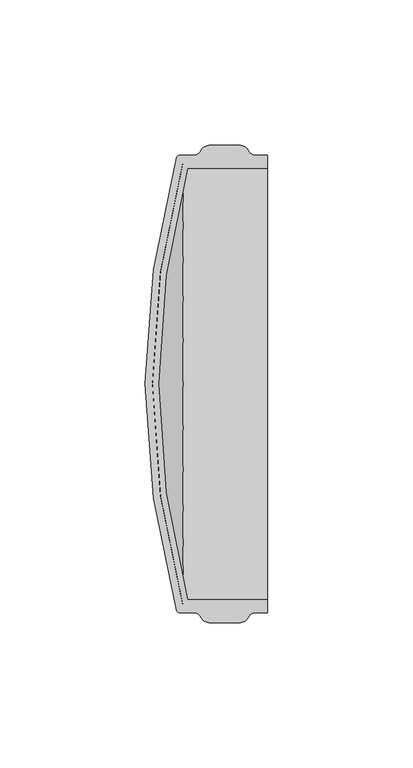
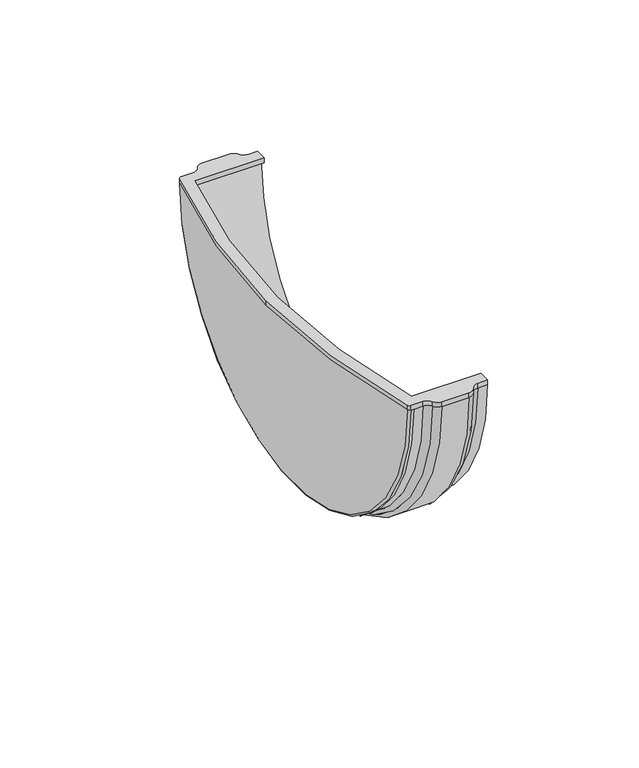
"""IFC4 building model written with IfcOpenShell, lengths in millimetres: proxy geometry, ↩ Заглушка желоба : ↩ Заглушка желоба."""

from ifc_helpers import new_model, si_unit, point, frame, origin, place, context, project, spatial, polyline, circle_curve, ellipse_curve, trimmed, source, transform, mapped, element, save
from ifc_brep_helpers import plane_surface, cylinder_surface, revolved_surface, advanced_brep


def generic_models_0d5aeb62(model_context):
    return source(origin(), model_context, "Body", "AdvancedBrep", [
        advanced_brep(
        [(-25.5074023, -78.6, 0.0), (-29.0, -78.6, 0.0), (-29.0, 78.6, 0.0), (-25.5074023, 78.6, 0.0), (-22.8037012, 80.3, 0.0), (-22.8037012, -80.3, 0.0), (-20.1, 82.0, 0.0), (-20.1, -82.0, 0.0), (-9.3443413, 82.0, 0.0), (-9.3443413, -82.0, 0.0), (-6.6406401, 80.3, 0.0), (-6.6406401, -80.3, 0.0), (-3.936939, 78.6, 0.0), (-3.936939, -78.6, 0.0), (-0.0443413, 78.6, 0.0), (-0.0443413, -78.6, 0.0), (-0.0443413, 78.6, 2.0), (-0.0443413, 74.1, 2.0), (-0.0443413, 74.1, 0.0), (-0.0443413, 76.1, 0.0), (-0.0443413, -76.1, 0.0), (-0.0443413, -74.1, 0.0), (-0.0443413, -74.1, 2.0), (-0.0443413, -78.6, 2.0), (-29.0, 76.1, 0.0), (-29.0, -76.1, 0.0), (-31.2572877, -77.8330313, 0.0), (-42.0295138, 0.0, 0.0), (-31.2572877, 77.8330313, 0.0), (-30.2504109, 78.6, 0.0), (-30.2504109, -78.6, 0.0), (-39.5258282, 0.0, 0.0), (-27.4693868, -74.1, 2.0), (-37.5257643, 0.0, 2.0), (-27.4693868, 74.1, 2.0), (-3.936939, 78.6, 2.0), (-6.6406401, 80.3, 2.0), (-9.3443413, 82.0, 2.0), (-20.1, 82.0, 2.0), (-22.8037012, 80.3, 2.0), (-25.5074023, 78.6, 2.0), (-30.2504109, 78.6, 2.0), (-31.2572877, 77.8330313, 2.0), (-42.0295138, 0.0, 2.0), (-31.2572877, -77.8330313, 2.0), (-30.2504109, -78.6, 2.0), (-25.5074023, -78.6, 2.0), (-22.8037012, -80.3, 2.0), (-20.1, -82.0, 2.0), (-9.3443413, -82.0, 2.0), (-6.6406401, -80.3, 2.0), (-3.936939, -78.6, 2.0), (-27.4693868, 74.1, 0.0), (-37.5257643, 0.0, 0.0), (-27.4693868, -74.1, 0.0)],
        [
            (0, 1),
            (1, 2, circle_curve(frame((-29.0, 0.0, 0.0), z_axis=(1.0, 0.0, 0.0), x_axis=(0.0, 1.0, 0.0)), 78.6)),
            (2, 3),
            (3, 0, circle_curve(frame((-25.5074023, 0.0, 0.0), z_axis=(-1.0, 0.0, 0.0), x_axis=(0.0, 1.0, 0.0)), 78.6)),
            (3, 4, circle_curve(frame((-25.5074023, 81.6, 0.0), z_axis=(0.0, 0.0, 1.0), x_axis=(1.0, 0.0, 0.0)), 3.0)),
            (4, 5, circle_curve(frame((-22.8037012, 0.0, 0.0), z_axis=(-1.0, 0.0, 0.0), x_axis=(0.0, 1.0, 0.0)), 80.3)),
            (5, 0, circle_curve(frame((-25.5074023, -81.6, 0.0), z_axis=(0.0, 0.0, 1.0), x_axis=(1.0, 0.0, 0.0)), 3.0)),
            (4, 6, circle_curve(frame((-20.1, 79.0, 0.0), z_axis=(0.0, 0.0, -1.0), x_axis=(1.0, 0.0, 0.0)), 3.0)),
            (6, 7, circle_curve(frame((-20.1, 0.0, 0.0), z_axis=(-1.0, 0.0, 0.0), x_axis=(0.0, 1.0, 0.0)), 82.0)),
            (7, 5, circle_curve(frame((-20.1, -79.0, 0.0), z_axis=(0.0, 0.0, -1.0), x_axis=(1.0, 0.0, 0.0)), 3.0)),
            (6, 8),
            (8, 9, circle_curve(frame((-9.3443413, 0.0, 0.0), z_axis=(-1.0, 0.0, 0.0), x_axis=(0.0, 1.0, 0.0)), 82.0)),
            (9, 7),
            (8, 10, circle_curve(frame((-9.3443413, 79.0, 0.0), z_axis=(0.0, 0.0, -1.0), x_axis=(-1.0, 0.0, 0.0)), 3.0)),
            (10, 11, circle_curve(frame((-6.6406401, 0.0, 0.0), z_axis=(-1.0, 0.0, 0.0), x_axis=(0.0, 1.0, 0.0)), 80.3)),
            (11, 9, circle_curve(frame((-9.3443413, -79.0, 0.0), z_axis=(0.0, 0.0, -1.0), x_axis=(-1.0, 0.0, 0.0)), 3.0)),
            (10, 12, circle_curve(frame((-3.936939, 81.6, 0.0), z_axis=(0.0, 0.0, 1.0), x_axis=(-1.0, 0.0, 0.0)), 3.0)),
            (12, 13, circle_curve(frame((-3.936939, 0.0, 0.0), z_axis=(-1.0, 0.0, 0.0), x_axis=(0.0, 1.0, 0.0)), 78.6)),
            (13, 11, circle_curve(frame((-3.936939, -81.6, 0.0), z_axis=(0.0, 0.0, 1.0), x_axis=(-1.0, 0.0, 0.0)), 3.0)),
            (12, 14),
            (14, 15, circle_curve(frame((-0.0443413, 0.0, 0.0), z_axis=(-1.0, 0.0, 0.0), x_axis=(0.0, 1.0, 0.0)), 78.6)),
            (15, 13),
            (14, 16),
            (16, 17),
            (17, 18),
            (18, 19),
            (19, 20, circle_curve(frame((-0.0443413, 0.0, 0.0), z_axis=(-1.0, 0.0, 0.0), x_axis=(0.0, 1.0, 0.0)), 76.1)),
            (20, 21),
            (21, 22),
            (22, 23),
            (23, 15),
            (19, 24),
            (24, 25, circle_curve(frame((-29.0, 0.0, 0.0), z_axis=(-1.0, 0.0, 0.0), x_axis=(0.0, 1.0, 0.0)), 76.1)),
            (25, 20),
            (26, 27, circle_curve(frame((257.964734, 1.8577595, 0.0), z_axis=(0.0, 0.0, -1.0), x_axis=(1.0, 0.0, 0.0)), 300.0)),
            (27, 28, circle_curve(frame((257.964734, -1.8577595, 0.0), z_axis=(0.0, 0.0, -1.0), x_axis=(1.0, 0.0, 0.0)), 300.0)),
            (28, 26, circle_curve(frame((-31.2572877, 0.0, 0.0), z_axis=(-1.0, 0.0, 0.0), x_axis=(0.0, 1.0, 0.0)), 77.8330313)),
            (28, 29, circle_curve(frame((-30.2504109, 77.5556015, 0.0), z_axis=(0.0, 0.0, -1.0), x_axis=(1.0, 0.0, 0.0)), 1.0443985)),
            (29, 30, circle_curve(frame((-30.2504109, 0.0, 0.0), z_axis=(-1.0, 0.0, 0.0), x_axis=(0.0, 1.0, 0.0)), 78.6)),
            (30, 26, circle_curve(frame((-30.2504109, -77.5556015, 0.0), z_axis=(0.0, 0.0, -1.0), x_axis=(1.0, 0.0, 0.0)), 1.0443985)),
            (29, 2),
            (1, 30),
            (24, 31, circle_curve(frame((257.964734, -2.3696848, 0.0), z_axis=(0.0, 0.0, 1.0), x_axis=(1.0, 0.0, 0.0)), 297.5)),
            (31, 25, circle_curve(frame((257.964734, 2.3696848, 0.0), z_axis=(0.0, 0.0, 1.0), x_axis=(1.0, 0.0, 0.0)), 297.5)),
            (22, 32),
            (32, 33, circle_curve(frame((257.964734, 2.3696848, 2.0), z_axis=(0.0, 0.0, -1.0), x_axis=(1.0, 0.0, 0.0)), 295.5)),
            (33, 34, circle_curve(frame((257.964734, -2.3696848, 2.0), z_axis=(0.0, 0.0, -1.0), x_axis=(1.0, 0.0, 0.0)), 295.5)),
            (34, 17),
            (16, 35),
            (35, 36, circle_curve(frame((-3.936939, 81.6, 2.0), z_axis=(0.0, 0.0, -1.0), x_axis=(1.0, 0.0, 0.0)), 3.0)),
            (36, 37, circle_curve(frame((-9.3443413, 79.0, 2.0), z_axis=(0.0, 0.0, 1.0), x_axis=(1.0, 0.0, 0.0)), 3.0)),
            (37, 38),
            (38, 39, circle_curve(frame((-20.1, 79.0, 2.0), z_axis=(0.0, 0.0, 1.0), x_axis=(1.0, 0.0, 0.0)), 3.0)),
            (39, 40, circle_curve(frame((-25.5074023, 81.6, 2.0), z_axis=(0.0, 0.0, -1.0), x_axis=(1.0, 0.0, 0.0)), 3.0)),
            (40, 41),
            (41, 42, circle_curve(frame((-30.2504109, 77.5556015, 2.0), z_axis=(0.0, 0.0, 1.0), x_axis=(1.0, 0.0, 0.0)), 1.0443985)),
            (42, 43, circle_curve(frame((257.964734, -1.8577595, 2.0), z_axis=(0.0, 0.0, 1.0), x_axis=(1.0, 0.0, 0.0)), 300.0)),
            (43, 44, circle_curve(frame((257.964734, 1.8577595, 2.0), z_axis=(0.0, 0.0, 1.0), x_axis=(1.0, 0.0, 0.0)), 300.0)),
            (44, 45, circle_curve(frame((-30.2504109, -77.5556015, 2.0), z_axis=(0.0, 0.0, 1.0), x_axis=(1.0, 0.0, 0.0)), 1.0443985)),
            (45, 46),
            (46, 47, circle_curve(frame((-25.5074023, -81.6, 2.0), z_axis=(0.0, 0.0, -1.0), x_axis=(1.0, 0.0, 0.0)), 3.0)),
            (47, 48, circle_curve(frame((-20.1, -79.0, 2.0), z_axis=(0.0, 0.0, 1.0), x_axis=(1.0, 0.0, 0.0)), 3.0)),
            (48, 49),
            (49, 50, circle_curve(frame((-9.3443413, -79.0, 2.0), z_axis=(0.0, 0.0, 1.0), x_axis=(1.0, 0.0, 0.0)), 3.0)),
            (50, 51, circle_curve(frame((-3.936939, -81.6, 2.0), z_axis=(0.0, 0.0, -1.0), x_axis=(1.0, 0.0, 0.0)), 3.0)),
            (51, 23),
            (18, 52),
            (52, 53, circle_curve(frame((257.964734, -2.3696848, 0.0), z_axis=(0.0, 0.0, 1.0), x_axis=(1.0, 0.0, 0.0)), 295.5)),
            (53, 54, circle_curve(frame((257.964734, 2.3696848, 0.0), z_axis=(0.0, 0.0, 1.0), x_axis=(1.0, 0.0, 0.0)), 295.5)),
            (54, 21),
            (51, 13),
            (50, 11),
            (49, 9),
            (48, 7),
            (47, 5),
            (46, 0),
            (45, 30),
            (44, 26),
            (43, 27),
            (42, 28),
            (41, 29),
            (40, 3),
            (39, 4),
            (38, 6),
            (37, 8),
            (36, 10),
            (35, 12),
            (34, 52),
            (33, 53),
            (32, 54),
        ],
        [
            cylinder_surface(frame((-14.7221706, 0.0, 0.0), z_axis=(1.0, 0.0, 0.0), x_axis=(0.0, 1.0, 0.0)), 78.6),
            revolved_surface(trimmed(ellipse_curve(frame((-25.5074023, 81.6, 0.0), z_axis=(0.0, 0.0, 1.0), x_axis=(1.0, 0.0, 0.0)), 3.0, 3.0), [point((-25.5074023, 78.6, 0.0))], [point((-22.8037012, 80.3, 0.0))], True, "CARTESIAN"), (-14.7221706, 0.0, 0.0), (1.0, 0.0, 0.0)),
            revolved_surface(trimmed(ellipse_curve(frame((-20.1, 79.0, 0.0), z_axis=(0.0, 0.0, -1.0), x_axis=(1.0, 0.0, 0.0)), 3.0, 3.0), [point((-22.8037012, 80.3, 0.0))], [point((-20.1, 82.0, 0.0))], True, "CARTESIAN"), (-14.7221706, 0.0, 0.0), (1.0, 0.0, 0.0)),
            cylinder_surface(frame((-14.7221706, 0.0, 0.0), z_axis=(1.0, 0.0, 0.0), x_axis=(0.0, 1.0, 0.0)), 82.0),
            revolved_surface(trimmed(ellipse_curve(frame((-9.3443413, 79.0, 0.0), z_axis=(0.0, 0.0, -1.0), x_axis=(-1.0, 0.0, 0.0)), 3.0, 3.0), [point((-9.3443413, 82.0, 0.0))], [point((-6.6406401, 80.3, 0.0))], True, "CARTESIAN"), (-14.7221706, 0.0, 0.0), (1.0, 0.0, 0.0)),
            revolved_surface(trimmed(ellipse_curve(frame((-3.936939, 81.6, 0.0), z_axis=(0.0, 0.0, 1.0), x_axis=(-1.0, 0.0, 0.0)), 3.0, 3.0), [point((-6.6406401, 80.3, 0.0))], [point((-3.936939, 78.6, 0.0))], True, "CARTESIAN"), (-14.7221706, 0.0, 0.0), (1.0, 0.0, 0.0)),
            plane_surface(frame((-0.0443413, 0.0, 0.0), z_axis=(1.0, 0.0, 0.0), x_axis=(0.0, 1.0, 0.0))),
            revolved_surface(polyline([(-0.04434129999999925, 76.1, 0.0), (-29.0, 76.1, 0.0)]), (-14.7221706, 0.0, 0.0), (1.0, 0.0, 0.0)),
            revolved_surface(trimmed(ellipse_curve(frame((257.964734, -1.8577595, 0.0), z_axis=(0.0, 0.0, -1.0), x_axis=(1.0, 0.0, 0.0)), 300.0, 300.0), [point((-42.0295138, 0.0, 0.0))], [point((-31.2572877, 77.8330313, 0.0))], True, "CARTESIAN"), (-42.0, 0.0, 0.0), (1.0, 0.0, 0.0)),
            revolved_surface(trimmed(ellipse_curve(frame((-30.2504109, 77.5556015, 0.0), z_axis=(0.0, 0.0, -1.0), x_axis=(1.0, 0.0, 0.0)), 1.0443985, 1.0443985), [point((-31.2572877, 77.8330313, 0.0))], [point((-30.2504109, 78.6, 0.0))], True, "CARTESIAN"), (-42.0, 0.0, 0.0), (1.0, 0.0, 0.0)),
            cylinder_surface(frame((-42.0, 0.0, 0.0), z_axis=(1.0, 0.0, 0.0), x_axis=(0.0, 1.0, 0.0)), 78.6),
            revolved_surface(trimmed(ellipse_curve(frame((257.964734, -2.3696848, 0.0), z_axis=(0.0, 0.0, 1.0), x_axis=(1.0, 0.0, 0.0)), 297.5, 297.5), [point((-29.0, 76.1, 0.0))], [point((-39.5258282, 0.0, 0.0))], True, "CARTESIAN"), (-42.0, 0.0, 0.0), (1.0, 0.0, 0.0)),
            plane_surface(frame((-0.0443413, -78.6, 2.0), z_axis=(0.0, 0.0, 1.0), x_axis=(-1.0, 0.0, 0.0))),
            plane_surface(frame((-0.0443413, -78.6, 0.0), z_axis=(0.0, 0.0, -1.0), x_axis=(1.0, 0.0, 0.0))),
            plane_surface(frame((-0.0443413, -78.6, 2.0), z_axis=(0.0, -1.0, 0.0), x_axis=(0.0, 0.0, -1.0))),
            revolved_surface(polyline([(-0.9369390000000002, -81.6, 0.0), (-0.9369390000000002, -81.6, 2.0)]), (-3.936939, -81.6, 0.0), (0.0, 0.0, -1.0)),
            cylinder_surface(frame((-9.3443413, -79.0, 0.0), z_axis=(0.0, 0.0, 1.0), x_axis=(1.0, 0.0, 0.0)), 3.0),
            plane_surface(frame((-9.3443413, -82.0, 2.0), z_axis=(0.0, -1.0, 0.0), x_axis=(0.0, 0.0, -1.0))),
            cylinder_surface(frame((-20.1, -79.0, 0.0), z_axis=(0.0, 0.0, 1.0), x_axis=(1.0, 0.0, 0.0)), 3.0),
            revolved_surface(polyline([(-22.5074023, -81.6, 0.0), (-22.5074023, -81.6, 2.0)]), (-25.5074023, -81.6, 0.0), (0.0, 0.0, -1.0)),
            plane_surface(frame((-25.5074023, -78.6, 2.0), z_axis=(0.0, -1.0, 0.0), x_axis=(0.0, 0.0, -1.0))),
            cylinder_surface(frame((-30.2504109, -77.5556015, 0.0), z_axis=(0.0, 0.0, 1.0), x_axis=(1.0, 0.0, 0.0)), 1.0443985),
            cylinder_surface(frame((257.964734, 1.8577595, 0.0), z_axis=(0.0, 0.0, 1.0), x_axis=(1.0, 0.0, 0.0)), 300.0),
            cylinder_surface(frame((257.964734, -1.8577595, 0.0), z_axis=(0.0, 0.0, 1.0), x_axis=(1.0, 0.0, 0.0)), 300.0),
            cylinder_surface(frame((-30.2504109, 77.5556015, 0.0), z_axis=(0.0, 0.0, 1.0), x_axis=(1.0, 0.0, 0.0)), 1.0443985),
            plane_surface(frame((-30.2504109, 78.6, 2.0), z_axis=(0.0, 1.0, 0.0), x_axis=(0.0, 0.0, -1.0))),
            revolved_surface(polyline([(-22.5074023, 81.6, 0.0), (-22.5074023, 81.6, 2.0)]), (-25.5074023, 81.6, 0.0), (0.0, 0.0, -1.0)),
            cylinder_surface(frame((-20.1, 79.0, 0.0), z_axis=(0.0, 0.0, 1.0), x_axis=(1.0, 0.0, 0.0)), 3.0),
            plane_surface(frame((-20.1, 82.0, 2.0), z_axis=(0.0, 1.0, 0.0), x_axis=(0.0, 0.0, -1.0))),
            cylinder_surface(frame((-9.3443413, 79.0, 0.0), z_axis=(0.0, 0.0, 1.0), x_axis=(1.0, 0.0, 0.0)), 3.0),
            revolved_surface(polyline([(-0.9369390000000002, 81.6, 0.0), (-0.9369390000000002, 81.6, 2.0)]), (-3.936939, 81.6, 0.0), (0.0, 0.0, -1.0)),
            plane_surface(frame((-3.936939, 78.6, 2.0), z_axis=(0.0, 1.0, 0.0), x_axis=(0.0, 0.0, -1.0))),
            plane_surface(frame((-0.0443413, 74.1, 2.0), z_axis=(0.0, -1.0, 0.0), x_axis=(0.0, 0.0, -1.0))),
            revolved_surface(polyline([(553.464734, -2.3696848, 0.0), (553.464734, -2.3696848, 2.0)]), (257.964734, -2.3696848, 0.0), (0.0, 0.0, -1.0)),
            revolved_surface(polyline([(553.464734, 2.3696848, 0.0), (553.464734, 2.3696848, 2.0)]), (257.964734, 2.3696848, 0.0), (0.0, 0.0, -1.0)),
            plane_surface(frame((-27.4693868, -74.1, 2.0), z_axis=(0.0, 1.0, 0.0), x_axis=(0.0, 0.0, -1.0))),
        ],
        [
            (0, [[1, 2, 3, 4]]),
            (1, [[5, 6, 7, -4]]),
            (2, [[8, 9, 10, -6]]),
            (3, [[11, 12, 13, -9]]),
            (4, [[14, 15, 16, -12]]),
            (5, [[17, 18, 19, -15]]),
            (0, [[20, 21, 22, -18]]),
            (6, [[23, 24, 25, 26, 27, 28, 29, 30, 31, -21]]),
            (7, [[32, 33, 34, -27]]),
            (8, [[35, 36, 37]]),
            (9, [[38, 39, 40, -37]]),
            (10, [[41, -2, 42, -39]]),
            (11, [[43, 44, -33]]),
            (12, [[-30, 45, 46, 47, 48, -24, 49, 50, 51, 52, 53, 54, 55, 56, 57, 58, 59, 60, 61, 62, 63, 64, 65, 66]]),
            (13, [[-28, -34, -44, -43, -32, -26, 67, 68, 69, 70]]),
            (14, [[71, -22, -31, -66]]),
            (15, [[72, -19, -71, -65]]),
            (16, [[73, -16, -72, -64]]),
            (17, [[74, -13, -73, -63]]),
            (18, [[75, -10, -74, -62]]),
            (19, [[76, -7, -75, -61]]),
            (20, [[77, -42, -1, -76, -60]]),
            (21, [[78, -40, -77, -59]]),
            (22, [[79, -35, -78, -58]]),
            (23, [[80, -36, -79, -57]]),
            (24, [[81, -38, -80, -56]]),
            (25, [[82, -3, -41, -81, -55]]),
            (26, [[83, -5, -82, -54]]),
            (27, [[84, -8, -83, -53]]),
            (28, [[85, -11, -84, -52]]),
            (29, [[86, -14, -85, -51]]),
            (30, [[87, -17, -86, -50]]),
            (31, [[-23, -20, -87, -49]]),
            (32, [[88, -67, -25, -48]]),
            (33, [[89, -68, -88, -47]]),
            (34, [[90, -69, -89, -46]]),
            (35, [[-29, -70, -90, -45]]),
        ],
    ),
    ])


if __name__ == "__main__":
    model = new_model("IFC4")
    model_context = context("Model", 3, world=origin())
    ifc_project = project(units=[si_unit("LENGTHUNIT", "METRE", prefix="MILLI")], contexts=[model_context])
    site = spatial("IfcSite", under=ifc_project)
    building = spatial("IfcBuilding", under=site)
    placement = place(None, origin())
    generic_models_shape = generic_models_0d5aeb62(model_context)
    element("IfcBuildingElementProxy", 1, Name="↩ Заглушка желоба : ↩ Заглушка желоба", ObjectType="↩ Заглушка желоба : ↩ Заглушка желоба", at=placement, inside=building, context=model_context, shape_type="MappedRepresentation", body=[
        mapped(generic_models_shape, transform((0.0, 0.0, 0.0), x_axis=(1.0, 0.0, 0.0), y_axis=(0.0, 1.0, 0.0), z_axis=(0.0, 0.0, 1.0))),
    ])
    save(model, "model.ifc")

# Revit data of these elements
# Type "↩ Заглушка желоба : ↩ Заглушка желоба"
#   Description = "Устанавливается на торцах желоба\r\nи направляет дождевую воду в сторону\r\nуклона к воронке."
#   Manufacturer = "ТехноНИКОЛЬ"
#   Model = "Комплектующие к водосточным системам"
#   URL = "https://tn-vodostok.ru/catalog/pvh/"
#   ADSK_Обозначение = "ТехноНИКОЛЬ"
#   ADSK_Наименование краткое = "Заглушка"
#   ADSK_Наименование = "Заглушка желоба"
#   ADSK_Масса_Текст = ""
#   ADSK_Марка = ""
#   ADSK_Код изделия = ""
#   ADSK_Завод-изготовитель = "ТехноНИКОЛЬ"
#   ADSK_Единица измерения = "шт."
#   ADSK_Группирование = "Комплектующие к водосточным системам"
#   ADSK_URL страницы изделия = "https://tn-vodostok.ru/catalog/pvh/"
#   ADSK_URL документации изделия = "https://tn-vodostok.ru/upload/iblock/c42/c427963cb77eb5c3c51f0cfb870e9e52.pdf"
#   Угол поворота кронштейна [instance default] = 0.00°
#   Длина пластины [instance default] = 0 mm
#   ADSK_Размер_Ширина = 164 mm
#   ADSK_Размер_Длина = 42 mm
#   ADSK_Размер_Высота = 82 mm
#   ADSK_Количество = 1
#   Видимость_Защитная решетка [instance default] = yes
#   Материал_Защитная решетка [instance default] = none
#   ADSK_Материал [instance default] = TN_Пластик_Коричневый_RAL8019
#   Default Elevation = 0
# Element 1 (IfcBuildingElementProxy, "↩ Заглушка желоба : ↩ Заглушка желоба")
#   Материал_Защитная решетка = TN_Пластик_Решетка_Коричневый_RAL8019
#   Materials on its faces: "TN_Пластик_Коричневый_RAL8019"
# Materials
#   "TN_Пластик_Коричневый_RAL8019": class "Типовые", colour RGB 61 54 53, transparency 0, Cost = 0
#   "TN_Пластик_Решетка_Коричневый_RAL8019": class "Типовые", colour RGB 61 54 53, transparency 0.25, Cost = 0
